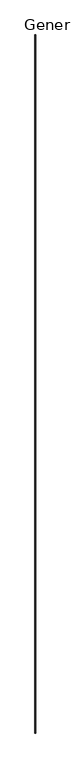
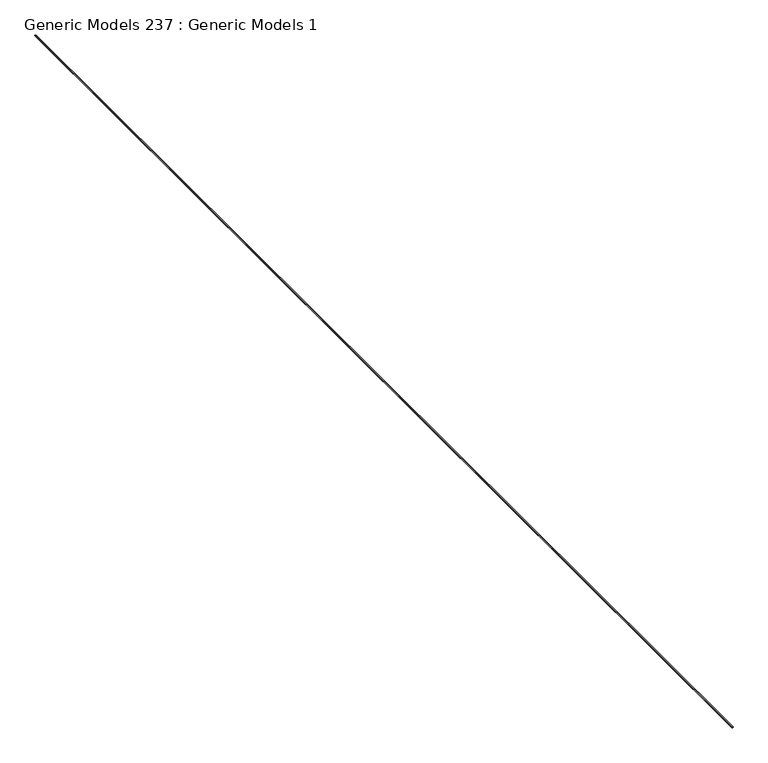
"""IFC4 building model written with IfcOpenShell, lengths in millimetres: proxy geometry, Generic Models 237 : Generic Models 1."""

from ifc_helpers import new_model, si_unit, point, frame, origin, place, context, project, spatial, polyline, circle_curve, ellipse_curve, trimmed, source, transform, mapped, element, save
from ifc_brep_helpers import plane_surface, cylinder_surface, revolved_surface, extruded_surface, advanced_brep


def generic_models_237_generic_models_1_2080604e(model_context):
    return source(origin(), model_context, "Body", "AdvancedBrep", [
        advanced_brep(
        [(31851.4669485, -6071.1841174, 129231.5872789), (31856.2294485, -6071.1841174, 129231.5872789), (31857.6570875, -6071.1841174, 129233.4932667), (31857.6570875, -6071.1841174, 129239.206291), (31856.2294485, -6071.1841174, 129241.1122789), (31851.4669485, -6071.1841174, 129241.1122789), (31851.4669485, 12978.8158826, 129231.5872789), (31851.4669485, 12978.8158826, 129241.1122789), (31856.2294485, 12978.8158826, 129241.1122789), (31857.6570875, 12978.8158826, 129239.206291), (31857.6570875, 12978.8158826, 129233.4932667), (31856.2294485, 12978.8158826, 129231.5872789)],
        [
            (0, 1),
            (1, 2, circle_curve(frame((31851.8573378, -6071.1841174, 129236.3497789), z_axis=(0.0, -1.0, 0.0), x_axis=(0.0, 0.0, -1.0)), 6.4650413)),
            (2, 3, ellipse_curve(frame((31863.3731985, -6071.1841174, 129236.3497789), z_axis=(0.0, -1.0, 0.0), x_axis=(-1.0, 0.0, 0.0)), 7.14375, 4.7625)),
            (3, 4, circle_curve(frame((31851.8573378, -6071.1841174, 129236.3497789), z_axis=(0.0, -1.0, 0.0), x_axis=(0.0, 0.0, -1.0)), 6.4650413)),
            (4, 5),
            (5, 0, circle_curve(frame((31847.0948378, -6071.1841174, 129236.3497789), z_axis=(0.0, 1.0, 0.0), x_axis=(0.0, 0.0, -1.0)), 6.4650413)),
            (6, 7, circle_curve(frame((31847.0948378, 12978.8158826, 129236.3497789), z_axis=(0.0, -1.0, 0.0), x_axis=(0.0, 0.0, -1.0)), 6.4650413)),
            (7, 8),
            (8, 9, circle_curve(frame((31851.8573378, 12978.8158826, 129236.3497789), z_axis=(0.0, 1.0, 0.0), x_axis=(0.0, 0.0, -1.0)), 6.4650413)),
            (9, 10, ellipse_curve(frame((31863.3731985, 12978.8158826, 129236.3497789), z_axis=(0.0, 1.0, 0.0), x_axis=(-1.0, 0.0, 0.0)), 7.14375, 4.7625)),
            (10, 11, circle_curve(frame((31851.8573378, 12978.8158826, 129236.3497789), z_axis=(0.0, 1.0, 0.0), x_axis=(0.0, 0.0, -1.0)), 6.4650413)),
            (11, 6),
            (2, 10),
            (9, 3),
            (5, 7),
            (6, 0),
            (4, 8),
            (1, 11),
        ],
        [
            plane_surface(frame((31851.4669485, -6071.1841174, 129241.1122789), z_axis=(0.0, -1.0, 0.0), x_axis=(-1.0, 0.0, 0.0))),
            plane_surface(frame((31851.4669485, 12978.8158826, 129241.1122789), z_axis=(0.0, 1.0, 0.0), x_axis=(-1.0, 0.0, 0.0))),
            extruded_surface(trimmed(ellipse_curve(frame((31863.3731985, 12978.8158826, 129236.3497789), z_axis=(0.0, -1.0, 0.0), x_axis=(-1.0, 0.0, 0.0)), 7.14375, 4.7625), [point((31857.6570875, 12978.8158826, 129233.4932667))], [point((31857.6570875, 12978.8158826, 129239.206291))], True, "CARTESIAN"), (0.0, -19050.0, 0.0), 19050.0),
            revolved_surface(polyline([(31847.0948378, 12978.8158826, 129229.88473759999), (31847.0948378, -6071.1841174, 129229.88473759999)]), (31847.0948378, -6071.1841174, 129236.3497789), (0.0, 1.0, 0.0)),
            plane_surface(frame((31856.2294485, -6071.1841174, 129241.1122789), z_axis=(0.0, 0.0, 1.0), x_axis=(0.0, 1.0, 0.0))),
            cylinder_surface(frame((31851.8573378, -6071.1841174, 129236.3497789), z_axis=(0.0, -1.0, 0.0), x_axis=(0.0, 0.0, -1.0)), 6.4650413),
            plane_surface(frame((31851.4669485, -6071.1841174, 129231.5872789), z_axis=(0.0, 0.0, -1.0), x_axis=(0.0, 1.0, 0.0))),
        ],
        [
            (0, [[1, 2, 3, 4, 5, 6]]),
            (1, [[7, 8, 9, 10, 11, 12]]),
            (2, [[-3, 13, -10, 14]]),
            (3, [[-6, 15, -7, 16]]),
            (4, [[-5, 17, -8, -15]]),
            (5, [[-4, -14, -9, -17]]),
            (5, [[-2, 18, -11, -13]]),
            (6, [[-1, -16, -12, -18]]),
        ],
    ),
    ])


if __name__ == "__main__":
    model = new_model("IFC4")
    model_context = context("Model", 3, world=origin())
    ifc_project = project(units=[si_unit("LENGTHUNIT", "METRE", prefix="MILLI")], contexts=[model_context])
    site = spatial("IfcSite", under=ifc_project)
    building = spatial("IfcBuilding", under=site)
    placement = place(None, origin())
    generic_models_237_generic_models_1_shape = generic_models_237_generic_models_1_2080604e(model_context)
    element("IfcBuildingElementProxy", 1, Name="Generic Models 237 : Generic Models 1", ObjectType="Generic Models 237 : Generic Models 1", at=placement, inside=building, context=model_context, shape_type="MappedRepresentation", body=[
        mapped(generic_models_237_generic_models_1_shape, transform((0.0, 0.0, 0.0), x_axis=(1.0, 0.0, 0.0), y_axis=(0.0, 1.0, 0.0), z_axis=(0.0, 0.0, 1.0))),
    ])
    save(model, "model.ifc")

# Revit data of these elements
# Element 1 (IfcBuildingElementProxy, "Generic Models 237 : Generic Models 1")
#   Materials on its faces: "_SEALANT AND BACKROD, IF NECESSARY"
# Materials
#   "_SEALANT AND BACKROD, IF NECESSARY": class "Generic", colour RGB 190 220 196, transparency 0, Cost = 0
